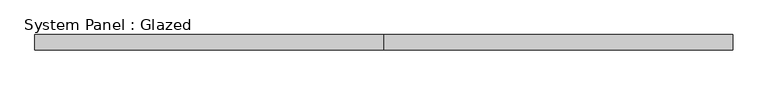
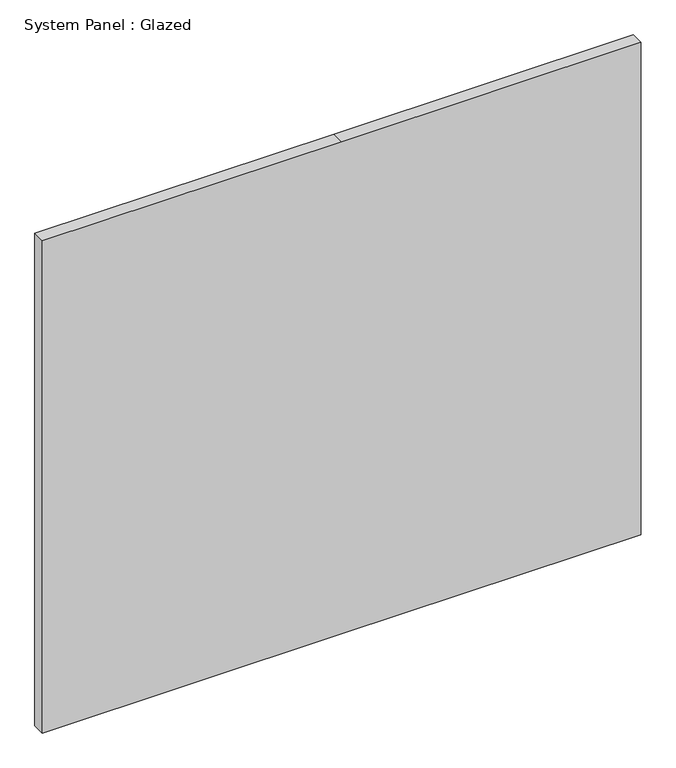
"""IFC4 building model written with IfcOpenShell, lengths in millimetres: plate geometry, System Panel : Glazed."""

from ifc_helpers import new_model, si_unit, frame, origin, place, context, project, spatial, polyline, outline, extrude, source, transform, mapped, element, save


def system_panel_glazed_239726b3(model_context):
    return source(origin(), model_context, "Body", "SweptSolid", [
        extrude(outline(polyline([(0.0, -1150.0), (0.0, 0.0), (0.0, 1150.0), (2000.0, 1150.0), (2000.0, 0.0), (2000.0, -1150.0), (0.0, -1150.0)])), frame((0.0, -25.0, 0.0), z_axis=(0.0, 1.0, 0.0), x_axis=(0.0, 0.0, 1.0)), (0.0, 0.0, 1.0), 50.0),
    ])


if __name__ == "__main__":
    model = new_model("IFC4")
    model_context = context("Model", 3, world=origin())
    ifc_project = project(units=[si_unit("LENGTHUNIT", "METRE", prefix="MILLI")], contexts=[model_context])
    site = spatial("IfcSite", under=ifc_project)
    building = spatial("IfcBuilding", under=site)
    placement = place(None, origin())
    system_panel_glazed_shape = system_panel_glazed_239726b3(model_context)
    element("IfcPlate", 1, ObjectType="System Panel : Glazed", at=placement, inside=building, context=model_context, shape_type="MappedRepresentation", body=[
        mapped(system_panel_glazed_shape, transform((0.0, 0.0, 0.0), x_axis=(1.0, 0.0, 0.0), y_axis=(0.0, 1.0, 0.0), z_axis=(0.0, 0.0, 1.0))),
    ])
    save(model, "model.ifc")

# Revit data of these elements
# Type "System Panel : Glazed"
#   Type Mark = "CW-GLASS"
# Element 1 (IfcPlate, "System Panel : Glazed")
#   Materials on its faces: "Glass_Clear"
# Materials
#   "Glass_Clear": class "Glass", colour RGB 128 128 255, transparency 0.8, Comments = "Rendering appearance not upgraded ", Cost = 0
